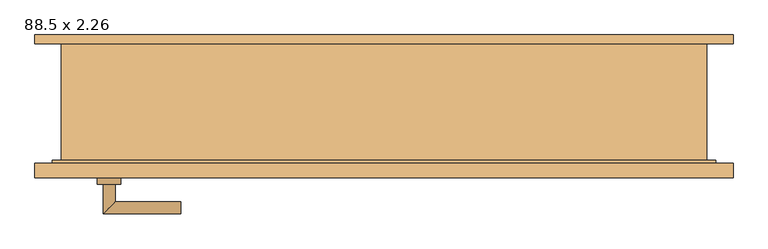
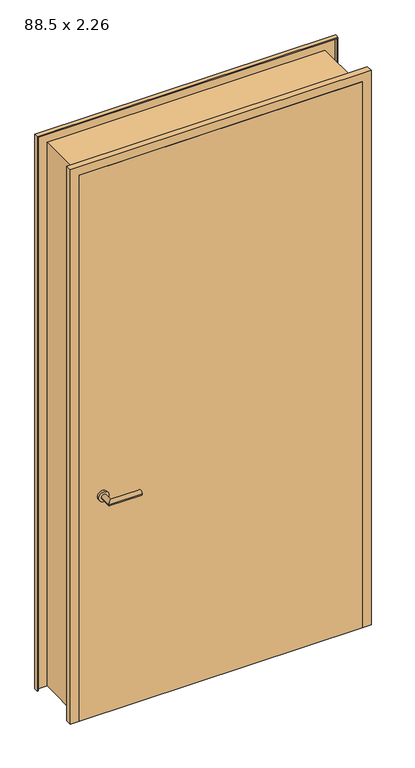
"""IFC4 building model written with IfcOpenShell, lengths in millimetres: door geometry, Drehflügel 1-flg - Stahlzarge : 88.5 x 2.26."""

from ifc_helpers import new_model, si_unit, point, frame, frame_2d, origin, place, context, project, spatial, polyline, circle_curve, ellipse_curve, trimmed, segment, composite_curve, outline, extrude, faceted_brep, source, transform, mapped, element, save
from ifc_brep_helpers import plane_surface, cylinder_surface, advanced_brep


def door_88_5_x_2_26_3adbfba5(model_context):
    return source(origin(), model_context, "Body", "SolidModel", [
        advanced_brep(
        [(-471.4, -89.4346141, 1000.0), (-451.4, -89.4346141, 1000.0), (-451.4, -39.4346141, 1000.0), (-471.4, -19.4346141, 1000.0), (-341.4, -19.4346141, 1000.0), (-341.4, -39.4346141, 1000.0)],
        [
            (0, 1, circle_curve(frame((-461.4, -89.4346141, 1000.0), z_axis=(0.0, -1.0, 0.0), x_axis=(1.0, 0.0, 0.0)), 10.0)),
            (1, 0, circle_curve(frame((-461.4, -89.4346141, 1000.0), z_axis=(0.0, -1.0, 0.0), x_axis=(1.0, 0.0, 0.0)), 10.0)),
            (1, 2),
            (2, 3, ellipse_curve(frame((-461.4, -29.4346141, 1000.0), z_axis=(-0.7071067811865385, -0.7071067811865565, 0.0), x_axis=(0.7071067811865563, -0.7071067811865386, 0.0)), 14.1421356, 10.0)),
            (3, 0),
            (3, 2, ellipse_curve(frame((-461.4, -29.4346141, 1000.0), z_axis=(-0.7071067811865385, -0.7071067811865565, 0.0), x_axis=(0.7071067811865563, -0.7071067811865386, 0.0)), 14.1421356, 10.0)),
            (4, 5, circle_curve(frame((-341.4, -29.4346141, 1000.0), z_axis=(1.0, 0.0, 0.0), x_axis=(0.0, -1.0, 0.0)), 10.0)),
            (5, 4, circle_curve(frame((-341.4, -29.4346141, 1000.0), z_axis=(1.0, 0.0, 0.0), x_axis=(0.0, -1.0, 0.0)), 10.0)),
            (2, 5),
            (4, 3),
        ],
        [
            plane_surface(frame((-461.4, -89.4346141, -287.7526403), z_axis=(0.0, -1.0, 0.0), x_axis=(0.0, 0.0, 1.0))),
            cylinder_surface(frame((-461.4, -89.4346141, 1000.0), z_axis=(0.0, -1.0, 0.0), x_axis=(1.0, 0.0, 0.0)), 10.0),
            plane_surface(frame((-341.4, -29.4346141, -287.7526403), z_axis=(1.0, 0.0, 0.0), x_axis=(0.0, 0.0, 1.0))),
            cylinder_surface(frame((-461.4, -29.4346141, 1000.0), z_axis=(-1.0, 0.0, 0.0), x_axis=(0.0, -1.0, 0.0)), 10.0),
        ],
        [
            (0, [[1, 2]]),
            (1, [[3, 4, 5, -2]]),
            (1, [[-5, 6, -3, -1]]),
            (2, [[7, 8]]),
            (3, [[9, -7, 10, -4]]),
            (3, [[-10, -8, -9, -6]]),
        ],
    ),
        advanced_brep(
        [(-451.4, -149.4346141, 1000.0), (-471.4, -149.4346141, 1000.0), (-471.4, -199.4346141, 1000.0), (-451.4, -179.4346141, 1000.0), (-341.4, -179.4346141, 1000.0), (-341.4, -199.4346141, 1000.0)],
        [
            (0, 1, circle_curve(frame((-461.4, -149.4346141, 1000.0), z_axis=(0.0, 1.0, 0.0), x_axis=(-1.0, 0.0, 0.0)), 10.0)),
            (1, 0, circle_curve(frame((-461.4, -149.4346141, 1000.0), z_axis=(0.0, 1.0, 0.0), x_axis=(-1.0, 0.0, 0.0)), 10.0)),
            (1, 2),
            (2, 3, ellipse_curve(frame((-461.4, -189.4346141, 1000.0), z_axis=(-0.7071067811865475, 0.7071067811865475, 0.0), x_axis=(0.7071067811865474, 0.7071067811865476, 0.0)), 14.1421356, 10.0)),
            (3, 0),
            (3, 2, ellipse_curve(frame((-461.4, -189.4346141, 1000.0), z_axis=(-0.7071067811865475, 0.7071067811865475, 0.0), x_axis=(0.7071067811865474, 0.7071067811865476, 0.0)), 14.1421356, 10.0)),
            (4, 5, circle_curve(frame((-341.4, -189.4346141, 1000.0), z_axis=(1.0, 0.0, 0.0), x_axis=(0.0, -1.0, 0.0)), 10.0)),
            (5, 4, circle_curve(frame((-341.4, -189.4346141, 1000.0), z_axis=(1.0, 0.0, 0.0), x_axis=(0.0, -1.0, 0.0)), 10.0)),
            (2, 5),
            (4, 3),
        ],
        [
            plane_surface(frame((-461.4, -149.4346141, -287.7526403), z_axis=(0.0, 1.0, 0.0), x_axis=(0.0, 0.0, 1.0))),
            cylinder_surface(frame((-461.4, -149.4346141, 1000.0), z_axis=(0.0, 1.0, 0.0), x_axis=(-1.0, 0.0, 0.0)), 10.0),
            plane_surface(frame((-341.4, -189.4346141, -287.7526403), z_axis=(1.0, 0.0, 0.0), x_axis=(0.0, 0.0, 1.0))),
            cylinder_surface(frame((-461.4, -189.4346141, 1000.0), z_axis=(-1.0, 0.0, 0.0), x_axis=(0.0, -1.0, 0.0)), 10.0),
        ],
        [
            (0, [[1, 2]]),
            (1, [[3, 4, 5, -2]]),
            (1, [[-5, 6, -3, -1]]),
            (2, [[7, 8]]),
            (3, [[9, -7, 10, -4]]),
            (3, [[-10, -8, -9, -6]]),
        ],
    ),
        extrude(outline(composite_curve([segment(trimmed(circle_curve(frame_2d((1000.0, -461.4)), 20.0), [point((1000.0, -481.4))], [point((1000.0, -441.4))], False, "CARTESIAN"), True, "CONTINUOUS"), segment(trimmed(circle_curve(frame_2d((1000.0, -461.4)), 20.0), [point((1000.0, -441.4))], [point((1000.0, -481.4))], False, "CARTESIAN"), True, "CONTINUOUS")], self_intersect=False)), frame((0.0, -89.4346141, 0.0), z_axis=(0.0, 1.0, 0.0), x_axis=(0.0, 0.0, 1.0)), (0.0, 0.0, 1.0), 10.0),
        extrude(outline(composite_curve([segment(trimmed(circle_curve(frame_2d((1000.0, -461.4)), 20.0), [point((1000.0, -481.4))], [point((1000.0, -441.4))], False, "CARTESIAN"), True, "CONTINUOUS"), segment(trimmed(circle_curve(frame_2d((1000.0, -461.4)), 20.0), [point((1000.0, -441.4))], [point((1000.0, -481.4))], False, "CARTESIAN"), True, "CONTINUOUS")], self_intersect=False)), frame((0.0, -149.4346141, 0.0), z_axis=(0.0, 1.0, 0.0), x_axis=(0.0, 0.0, 1.0)), (0.0, 0.0, 1.0), 10.0),
        extrude(outline(polyline([(551.4, -114.4346141), (551.4, -139.4346141), (-551.4, -139.4346141), (-551.4, -114.4346141), (551.4, -114.4346141)])), frame((0.0, 0.0, 100.0), z_axis=(0.0, 0.0, 1.0), x_axis=(1.0, 0.0, 0.0)), (0.0, 0.0, 1.0), 2250.0),
        faceted_brep([(585.8603207, 100.5653859, 100.0), (585.8603207, 85.5653859, 100.0), (580.8603207, 85.5653859, 100.0), (580.8603207, 95.5653859, 100.0), (541.4, 95.5653859, 100.0), (541.4, -109.4346141, 100.0), (556.4, -109.4346141, 100.0), (556.4, -134.4346141, 100.0), (580.8603207, -134.4346141, 100.0), (580.8603207, -114.4346141, 100.0), (585.8603207, -114.4346141, 100.0), (585.8603207, -139.4346141, 100.0), (551.4, -139.4346141, 100.0), (551.4, -114.4346141, 100.0), (536.4, -114.4346141, 100.0), (536.4, 100.5653859, 100.0), (536.4, 100.5653859, 2335.0), (-536.4, 100.5653859, 2335.0), (-536.4, 100.5653859, 100.0), (-585.8603207, 100.5653859, 100.0), (-585.8603207, 100.5653859, 2384.4603207), (585.8603207, 100.5653859, 2384.4603207), (536.4, -114.4346141, 2335.0), (551.4, -114.4346141, 2350.0), (-551.4, -114.4346141, 2350.0), (-551.4, -114.4346141, 100.0), (-536.4, -114.4346141, 100.0), (-536.4, -114.4346141, 2335.0), (551.4, -139.4346141, 2350.0), (585.8603207, -139.4346141, 2384.4603207), (-585.8603207, -139.4346141, 2384.4603207), (-585.8603207, -139.4346141, 100.0), (-551.4, -139.4346141, 100.0), (-551.4, -139.4346141, 2350.0), (585.8603207, -114.4346141, 2384.4603207), (580.8603207, -114.4346141, 2379.4603207), (-580.8603207, -114.4346141, 2379.4603207), (-580.8603207, -114.4346141, 100.0), (-585.8603207, -114.4346141, 100.0), (-585.8603207, -114.4346141, 2384.4603207), (580.8603207, -134.4346141, 2379.4603207), (556.4, -134.4346141, 2355.0), (-556.4, -134.4346141, 2355.0), (-556.4, -134.4346141, 100.0), (-580.8603207, -134.4346141, 100.0), (-580.8603207, -134.4346141, 2379.4603207), (556.4, -109.4346141, 2355.0), (541.4, -109.4346141, 2340.0), (-541.4, -109.4346141, 2340.0), (-541.4, -109.4346141, 100.0), (-556.4, -109.4346141, 100.0), (-556.4, -109.4346141, 2355.0), (541.4, 95.5653859, 2340.0), (580.8603207, 95.5653859, 2379.4603207), (-580.8603207, 95.5653859, 2379.4603207), (-580.8603207, 95.5653859, 100.0), (-541.4, 95.5653859, 100.0), (-541.4, 95.5653859, 2340.0), (580.8603207, 85.5653859, 2379.4603207), (585.8603207, 85.5653859, 2384.4603207), (-585.8603207, 85.5653859, 2384.4603207), (-585.8603207, 85.5653859, 100.0), (-580.8603207, 85.5653859, 100.0), (-580.8603207, 85.5653859, 2379.4603207)], [[[0, 1, 2, 3, 4, 5, 6, 7, 8, 9, 10, 11, 12, 13, 14, 15]], [[15, 16, 17, 18, 19, 20, 21, 0]], [[14, 22, 16, 15]], [[13, 23, 24, 25, 26, 27, 22, 14]], [[12, 28, 23, 13]], [[11, 29, 30, 31, 32, 33, 28, 12]], [[10, 34, 29, 11]], [[9, 35, 36, 37, 38, 39, 34, 10]], [[8, 40, 35, 9]], [[7, 41, 42, 43, 44, 45, 40, 8]], [[6, 46, 41, 7]], [[5, 47, 48, 49, 50, 51, 46, 6]], [[4, 52, 47, 5]], [[3, 53, 54, 55, 56, 57, 52, 4]], [[2, 58, 53, 3]], [[1, 59, 60, 61, 62, 63, 58, 2]], [[0, 21, 59, 1]], [[20, 19, 61, 60]], [[19, 18, 26, 25, 32, 31, 38, 37, 44, 43, 50, 49, 56, 55, 62, 61]], [[27, 26, 18, 17]], [[33, 32, 25, 24]], [[39, 38, 31, 30]], [[45, 44, 37, 36]], [[51, 50, 43, 42]], [[57, 56, 49, 48]], [[63, 62, 55, 54]], [[22, 27, 17, 16]], [[28, 33, 24, 23]], [[34, 39, 30, 29]], [[40, 45, 36, 35]], [[46, 51, 42, 41]], [[52, 57, 48, 47]], [[58, 63, 54, 53]], [[21, 20, 60, 59]]]),
    ])


if __name__ == "__main__":
    model = new_model("IFC4")
    model_context = context("Model", 3, world=origin())
    ifc_project = project(units=[si_unit("LENGTHUNIT", "METRE", prefix="MILLI")], contexts=[model_context])
    site = spatial("IfcSite", under=ifc_project)
    building = spatial("IfcBuilding", under=site)
    placement = place(None, origin())
    door_88_5_x_2_26_shape = door_88_5_x_2_26_3adbfba5(model_context)
    element("IfcDoor", 1, ObjectType="Drehflügel 1-flg - Stahlzarge : 88.5 x 2.26", at=placement, inside=building, context=model_context, shape_type="MappedRepresentation", body=[
        mapped(door_88_5_x_2_26_shape, transform((0.0, 0.0, 0.0), x_axis=(1.0, 0.0, 0.0), y_axis=(0.0, 1.0, 0.0), z_axis=(0.0, 0.0, 1.0))),
    ])
    save(model, "model.ifc")

# Revit data of these elements
# Type "Drehflügel 1-flg - Stahlzarge : 88.5 x 2.26"
#   Construction Type Id = "MDOOR"
#   Type Mark = "20"
#   Operation = "SingleSwingRight"
#   Keynote = "16.03"
#   Analytic Construction = "Metall"
#   Thermal Resistance (R) = 0.270117 (m²·K)/W
#   Heat Transfer Coefficient (U) = 3.7021 W/(m²·K)
#   Rough Width = 1.1228 m
#   Rough Height [instance default] = 2.360 m
#   Höhe Türgriff [instance default] = 0.900 m
#   Height = 2.260 m
#   Fußbodenaufbau [instance default] = 0.100 m
#   Width = 1.1228 m
#   Sichtbarkeit Sturzlinien [instance default] = yes
#   Türgriff auswählen [instance default] = element 221079
#   Türgriff [instance default] = none
#   Türflügel [instance default] = none
#   Rahmen/Pfosten [instance default] = Metall - Lackiert - Grau
#   Visual Light Transmittance = 0
#   Solar Heat Gain Coefficient = 0
#   Function = (empty or 0)
#   Wall Closure = (empty or 0)
# Element 1 (IfcDoor, "Drehflügel 1-flg - Stahlzarge : 88.5 x 2.26")
#   Materials on its faces: "Metall - Lackiert - Grau", "Metall - Chrom", "Holz - Birke"
# Materials
#   "Metall - Lackiert - Grau": class "Farbe 1", colour RGB 98 98 98, transparency 0, Cost = 0
#   "Metall - Chrom": class "Metall", colour RGB 247 247 247, transparency 0, Cost = 0
#   "Holz - Birke": class "Holz", colour RGB 213 164 103, transparency 0, Cost = 0
